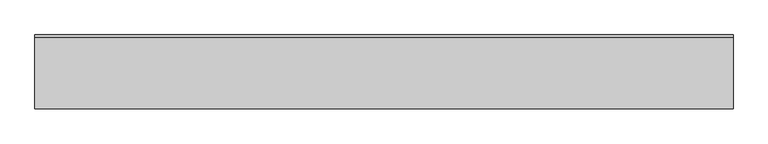
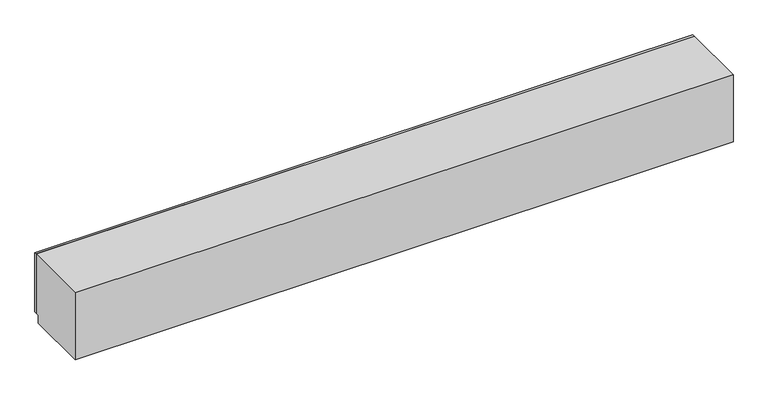
"""IFC4 building model written with IfcOpenShell, lengths in millimetres: furniture geometry, OD_CW_Base Cabinet : OD_CW_Base Cabinet."""

from ifc_helpers import new_model, si_unit, frame, origin, place, context, project, spatial, polyline, outline, extrude, source, transform, mapped, element, save


def furniture_5b6d99a9(model_context):
    return source(origin(), model_context, "Body", "SweptSolid", [
        extrude(outline(polyline([(18.7377049, 228.6), (18.7377049, 254.0), (8167.5056128, 254.0), (8167.5056128, 228.6), (18.7377049, 228.6)])), frame((0.0, 0.0, 101.6), z_axis=(0.0, 0.0, 1.0), x_axis=(1.0, 0.0, 0.0)), (0.0, 0.0, 1.0), 774.7),
        extrude(outline(polyline([(228.6, 876.3), (228.6, 101.6), (177.8, 101.6), (177.8, 0.0), (-609.6, 0.0), (-609.6, 876.3), (228.6, 876.3)])), frame((18.7377049, 0.0, 0.0), z_axis=(1.0, 0.0, 0.0), x_axis=(0.0, 1.0, 0.0)), (0.0, 0.0, 1.0), 8148.7679079),
    ])


if __name__ == "__main__":
    model = new_model("IFC4")
    model_context = context("Model", 3, world=origin())
    ifc_project = project(units=[si_unit("LENGTHUNIT", "METRE", prefix="MILLI")], contexts=[model_context])
    site = spatial("IfcSite", under=ifc_project)
    building = spatial("IfcBuilding", under=site)
    placement = place(None, origin())
    furniture_shape = furniture_5b6d99a9(model_context)
    element("IfcFurniture", 1, ObjectType="OD_CW_Base Cabinet : OD_CW_Base Cabinet", at=placement, inside=building, context=model_context, shape_type="MappedRepresentation", body=[
        mapped(furniture_shape, transform((0.0, 0.0, 0.0), x_axis=(1.0, 0.0, 0.0), y_axis=(0.0, 1.0, 0.0), z_axis=(0.0, 0.0, 1.0))),
    ])
    save(model, "model.ifc")

# Revit data of these elements
# Type "OD_CW_Base Cabinet : OD_CW_Base Cabinet"
#   OD_CW_Width [instance default] = 2' - 10"
#   OD_CW_Length [instance default] = 8' - 0"
#   OD_CW_Height [instance default] = 2' - 3"
#   Depth = 2' - 0"
#   Height = 3' - 0"
#   Width = 4' - 0"
#   OD_CW_Material_Front Panel [instance default] = none
#   OD_CW_Material_Body [instance default] = none
# Element 1 (IfcFurniture, "OD_CW_Base Cabinet : OD_CW_Base Cabinet")
#   OD_CW_Length = 26' - 8.81763"
#   OD_CW_Height = 2' - 10 1/2"
#   OD_CW_Material_Front Panel = WOOD-OAKFIRE
#   OD_CW_Material_Body = WOOD-OAKFIRE
#   Materials on its faces: "WOOD-OAKFIRE"
# Materials
#   "WOOD-OAKFIRE": class "Wood", colour RGB 198 202 183, transparency 0, Description = "Generic wood", Cost = 0
